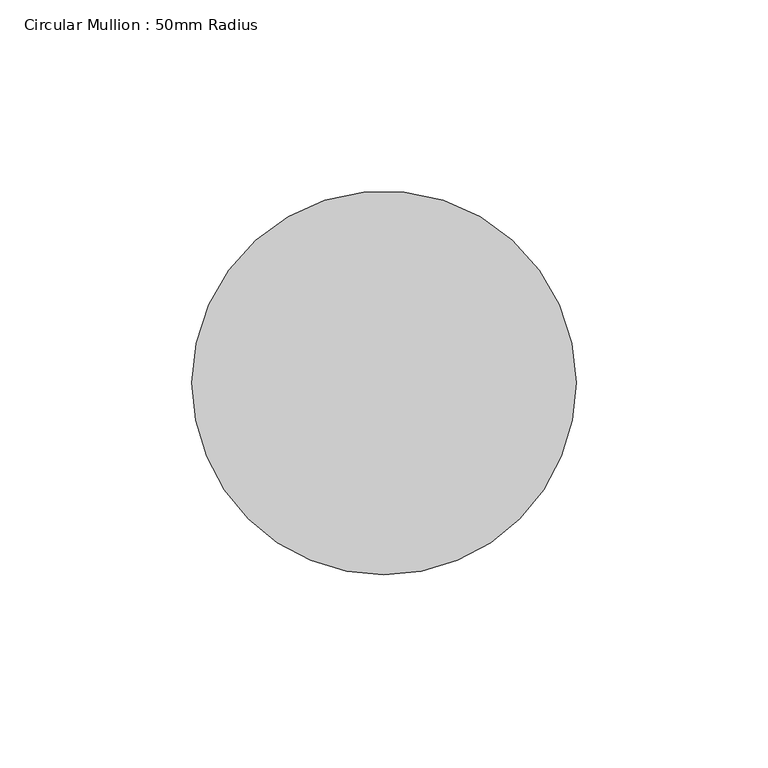
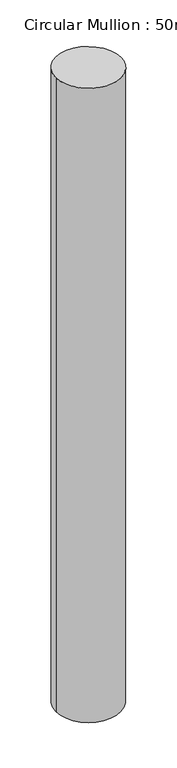
"""IFC4 building model written with IfcOpenShell, lengths in millimetres: member geometry, Circular Mullion : 50mm Radius."""

from ifc_helpers import new_model, si_unit, frame, origin, place, context, project, spatial, ellipse_curve, source, transform, mapped, element, save
from ifc_brep_helpers import plane_surface, cylinder_surface, advanced_brep


def circular_mullion_50mm_radius_f27c6aee(model_context):
    return source(origin(), model_context, "Body", "AdvancedBrep", [
        advanced_brep(
        [(-100.0, 0.0, 1.4978034), (0.0, 0.0, 0.0), (0.0, 0.0, -1028.7324588), (-100.0, 0.0, -1030.2579834)],
        [
            (0, 1, ellipse_curve(frame((-50.0, 0.0, 0.7489017), z_axis=(-0.014974646528253375, -0.015102099623456352, -0.9997738176949411), x_axis=(-0.7039447706942895, -0.7099362269672411, 0.02126766211134417)), 50.0113117, 50.0)),
            (1, 2),
            (2, 3, ellipse_curve(frame((-50.0, 0.0, -1029.4952211), z_axis=(-0.015251666192653642, -0.015381477073970836, 0.999765370895277), x_axis=(0.70393882326865, 0.7099302289214898, 0.021661097816809437)), 50.0117342, 50.0)),
            (3, 0),
            (1, 0, ellipse_curve(frame((-50.0, 0.0, 0.7489017), z_axis=(-0.014974646528253375, -0.015102099623456352, -0.9997738176949411), x_axis=(-0.7039447706942895, -0.7099362269672411, 0.02126766211134417)), 50.0113117, 50.0)),
            (3, 2, ellipse_curve(frame((-50.0, 0.0, -1029.4952211), z_axis=(-0.015251666192653642, -0.015381477073970836, 0.999765370895277), x_axis=(0.70393882326865, 0.7099302289214898, 0.021661097816809437)), 50.0117342, 50.0)),
        ],
        [
            cylinder_surface(frame((-50.0, 0.0, 0.0), z_axis=(0.0, 0.0, 1.0), x_axis=(1.0, 0.0, 0.0)), 50.0),
            plane_surface(frame((-216.4375163, 214.6109073, 0.0), z_axis=(0.014974646528253375, 0.015102099623456352, 0.9997738176949411), x_axis=(0.7039447706942903, 0.7099362269672399, -0.021267662111358908))),
            plane_surface(frame((-216.4375163, 214.6109073, -1028.7324588), z_axis=(0.015251666192653645, 0.01538147707397084, -0.9997653708952772), x_axis=(0.7039388232686501, 0.70993022892149, 0.0216610978168057))),
        ],
        [
            (0, [[1, 2, 3, 4]]),
            (0, [[5, -4, 6, -2]]),
            (1, [[-1, -5]]),
            (2, [[-6, -3]]),
        ],
    ),
    ])


if __name__ == "__main__":
    model = new_model("IFC4")
    model_context = context("Model", 3, world=origin())
    ifc_project = project(units=[si_unit("LENGTHUNIT", "METRE", prefix="MILLI")], contexts=[model_context])
    site = spatial("IfcSite", under=ifc_project)
    building = spatial("IfcBuilding", under=site)
    placement = place(None, origin())
    circular_mullion_50mm_radius_shape = circular_mullion_50mm_radius_f27c6aee(model_context)
    element("IfcMember", 1, ObjectType="Circular Mullion : 50mm Radius", at=placement, inside=building, context=model_context, shape_type="MappedRepresentation", body=[
        mapped(circular_mullion_50mm_radius_shape, transform((0.0, 0.0, 0.0), x_axis=(1.0, 0.0, 0.0), y_axis=(0.0, 1.0, 0.0), z_axis=(0.0, 0.0, 1.0))),
    ])
    save(model, "model.ifc")

# Revit data of these elements
# Type "Circular Mullion : 50mm Radius"
#   built-in parameter 1007350 = 0.164042 (stored number, unit not read)
# Element 1 (IfcMember, "Circular Mullion : 50mm Radius")
#   Materials on its faces: "Aluminium"
# Materials
#   "Aluminium": class "Metal", colour RGB 247 247 247, transparency 0, Description = "Aluminium 6061", Cost = 0
